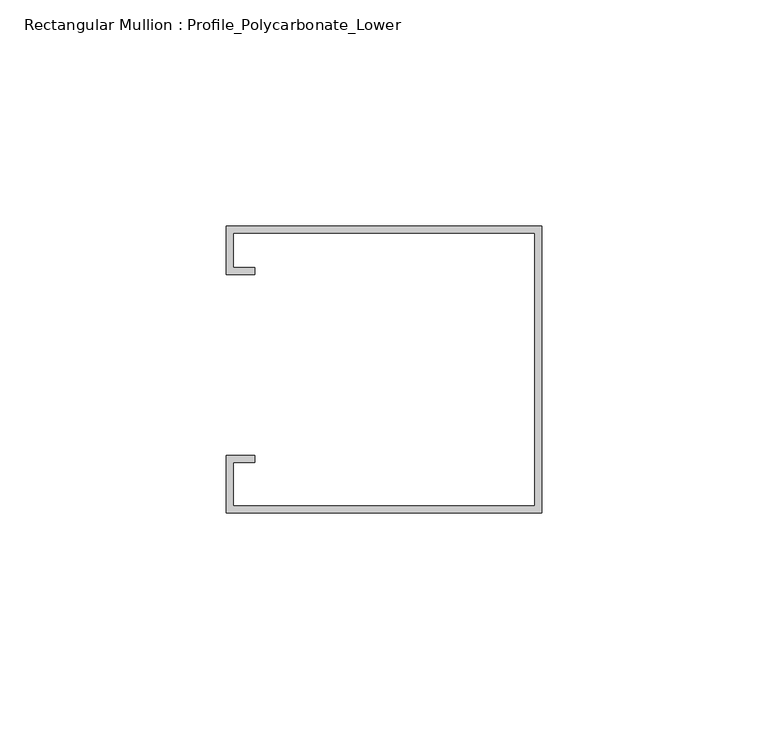
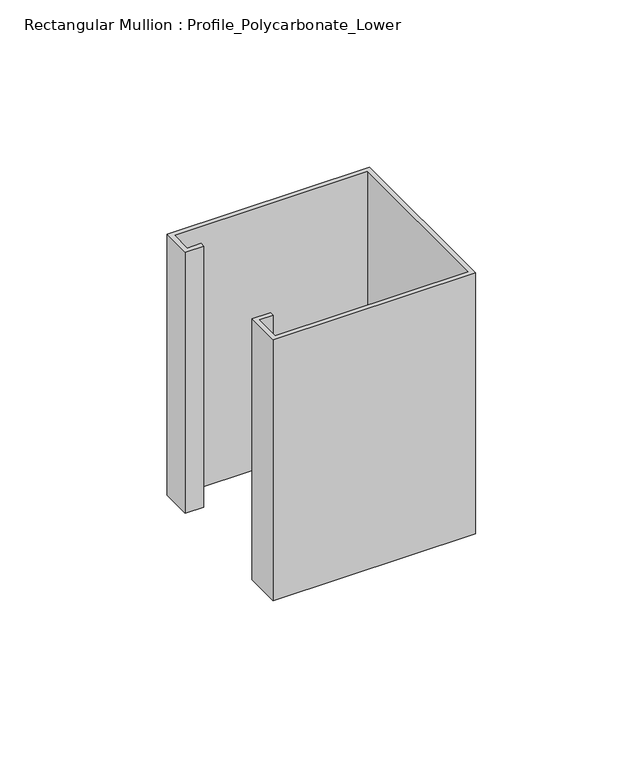
"""IFC4 building model written with IfcOpenShell, lengths in millimetres: member geometry, Rectangular Mullion : Profile_Polycarbonate_Lower."""

from ifc_helpers import new_model, si_unit, frame, origin, place, context, project, spatial, polyline, outline, extrude, source, transform, mapped, element, save


def rectangular_mullion_profile_polycarbonate_lower_993174bd(model_context):
    return source(origin(), model_context, "Body", "SweptSolid", [
        extrude(outline(polyline([(0.0, -32.7), (-69.85, -32.7), (-69.85, -20.0), (-63.5, -20.0), (-63.5, -21.5875), (-68.2625, -21.5875), (-68.2625, -31.1125), (-1.5875, -31.1125), (-1.5875, 29.2125), (-68.2625, 29.2125), (-68.2625, 21.5875), (-63.5, 21.5875), (-63.5, 20.0), (-69.85, 20.0), (-69.85, 30.8), (0.0, 30.8), (0.0, -32.7)])), frame((0.0, 0.0, -95.25), z_axis=(0.0, 0.0, 1.0), x_axis=(1.0, 0.0, 0.0)), (0.0, 0.0, 1.0), 95.25),
    ])


if __name__ == "__main__":
    model = new_model("IFC4")
    model_context = context("Model", 3, world=origin())
    ifc_project = project(units=[si_unit("LENGTHUNIT", "METRE", prefix="MILLI")], contexts=[model_context])
    site = spatial("IfcSite", under=ifc_project)
    building = spatial("IfcBuilding", under=site)
    placement = place(None, origin())
    rectangular_mullion_profile_polycarbonate_lower_shape = rectangular_mullion_profile_polycarbonate_lower_993174bd(model_context)
    element("IfcMember", 1, ObjectType="Rectangular Mullion : Profile_Polycarbonate_Lower", at=placement, inside=building, context=model_context, shape_type="MappedRepresentation", body=[
        mapped(rectangular_mullion_profile_polycarbonate_lower_shape, transform((0.0, 0.0, 0.0), x_axis=(1.0, 0.0, 0.0), y_axis=(0.0, 1.0, 0.0), z_axis=(0.0, 0.0, 1.0))),
    ])
    save(model, "model.ifc")

# Revit data of these elements
# Type "Rectangular Mullion : Profile_Polycarbonate_Lower"
#   built-in parameter 1007322 = 0.208333 (stored number, unit not read)
#   built-in parameter 1007321 = 0 (stored number, unit not read)
#   built-in parameter 1007320 = 0.00520833 (stored number, unit not read)
# Element 1 (IfcMember, "Rectangular Mullion : Profile_Polycarbonate_Lower")
#   Materials on its faces: "GALVANIZED UNISTRUT P5500, 1 5/8\" X 2 7/16\" OR ALUM. CHANNEL"
# Materials
#   "GALVANIZED UNISTRUT P5500, 1 5/8\" X 2 7/16\" OR ALUM. CHANNEL": class "Metal", colour RGB 244 244 244, transparency 0, Description = "Aluminum 6061", Cost = 0
